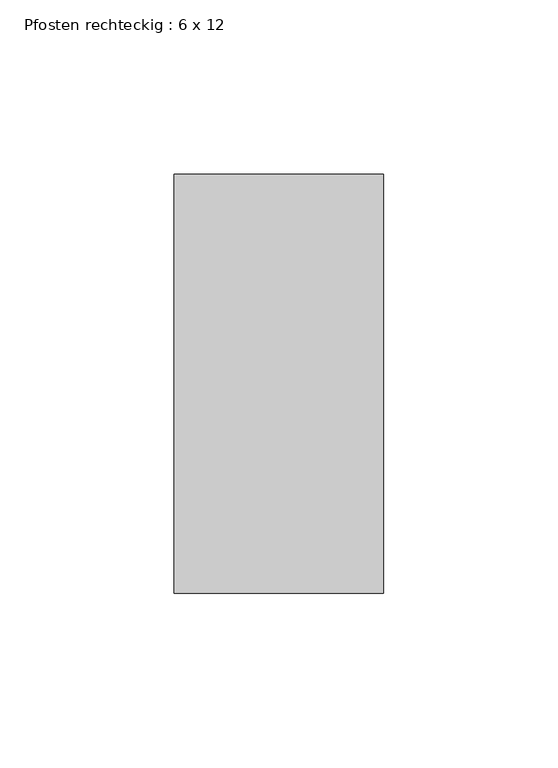
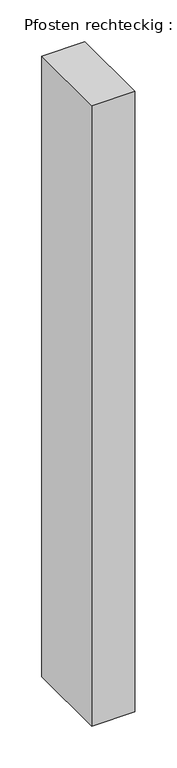
"""IFC4 building model written with IfcOpenShell, lengths in millimetres: member geometry, Pfosten rechteckig : 6 x 12."""

from ifc_helpers import new_model, si_unit, frame, origin, place, context, project, spatial, polyline, outline, extrude, source, transform, mapped, element, save


def pfosten_rechteckig_6_x_12_6c98ebb7(model_context):
    return source(origin(), model_context, "Body", "SweptSolid", [
        extrude(outline(polyline([(0.0, 60.0), (0.0, -60.0), (-60.0, -60.0), (-60.0, 60.0), (0.0, 60.0)])), frame((0.0, 0.0, -908.9641123), z_axis=(0.0, 0.0, 1.0), x_axis=(1.0, 0.0, 0.0)), (0.0, 0.0, 1.0), 908.9641123),
    ])


if __name__ == "__main__":
    model = new_model("IFC4")
    model_context = context("Model", 3, world=origin())
    ifc_project = project(units=[si_unit("LENGTHUNIT", "METRE", prefix="MILLI")], contexts=[model_context])
    site = spatial("IfcSite", under=ifc_project)
    building = spatial("IfcBuilding", under=site)
    placement = place(None, origin())
    pfosten_rechteckig_6_x_12_shape = pfosten_rechteckig_6_x_12_6c98ebb7(model_context)
    element("IfcMember", 1, ObjectType="Pfosten rechteckig : 6 x 12", at=placement, inside=building, context=model_context, shape_type="MappedRepresentation", body=[
        mapped(pfosten_rechteckig_6_x_12_shape, transform((0.0, 0.0, 0.0), x_axis=(1.0, 0.0, 0.0), y_axis=(0.0, 1.0, 0.0), z_axis=(0.0, 0.0, 1.0))),
    ])
    save(model, "model.ifc")

# Revit data of these elements
# Type "Pfosten rechteckig : 6 x 12"
#   built-in parameter 1007304 = 0.393701 (stored number, unit not read)
#   built-in parameter 1007301 = 0.0984252 (stored number, unit not read)
#   built-in parameter 1007300 = 0.0984252 (stored number, unit not read)
# Element 1 (IfcMember, "Pfosten rechteckig : 6 x 12")
#   Materials on its faces: "Metall - verzinkt"
# Materials
#   "Metall - verzinkt": class "Allgemeines", colour RGB 200 200 200, transparency 0, Cost = 0
